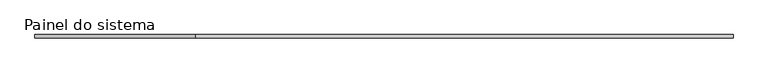
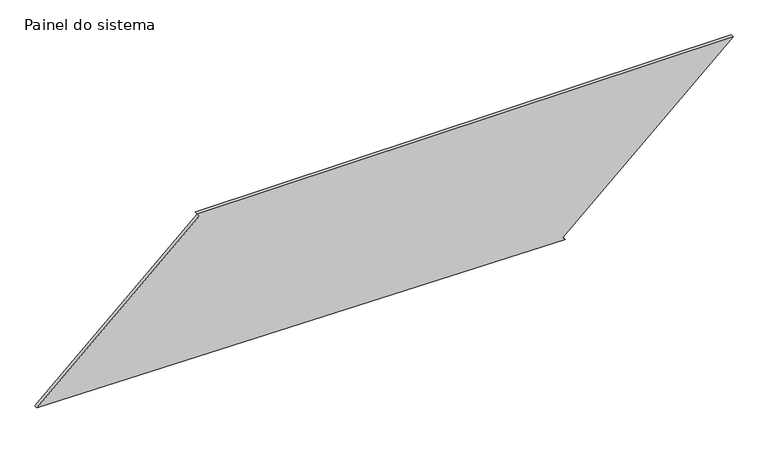
"""IFC4 building model written with IfcOpenShell, lengths in millimetres: plate geometry, Painel do sistema : Envidraçado."""

from ifc_helpers import new_model, si_unit, frame, origin, place, context, project, spatial, polyline, outline, extrude, source, transform, mapped, element, save


def painel_do_sistema_f254071a(model_context):
    return source(origin(), model_context, "Body", "SweptSolid", [
        extrude(outline(polyline([(0.0, 1281.7749259), (18.5968466, 1265.066925), (1106.0483241, 2475.4551949), (1106.0483241, -1336.534264), (1087.4514775, -1319.8262631), (49.1975382, -2475.4551949), (0.0, 1281.7749259)])), frame((0.0, 24.5, 0.0), z_axis=(0.0, 1.0, 0.0), x_axis=(0.0, 0.0, 1.0)), (0.0, 0.0, 1.0), 25.0),
    ])


if __name__ == "__main__":
    model = new_model("IFC4")
    model_context = context("Model", 3, world=origin())
    ifc_project = project(units=[si_unit("LENGTHUNIT", "METRE", prefix="MILLI")], contexts=[model_context])
    site = spatial("IfcSite", under=ifc_project)
    building = spatial("IfcBuilding", under=site)
    placement = place(None, origin())
    painel_do_sistema_shape = painel_do_sistema_f254071a(model_context)
    element("IfcPlate", 1, ObjectType="Painel do sistema : Envidraçado", at=placement, inside=building, context=model_context, shape_type="MappedRepresentation", body=[
        mapped(painel_do_sistema_shape, transform((0.0, 0.0, 0.0), x_axis=(1.0, 0.0, 0.0), y_axis=(0.0, 1.0, 0.0), z_axis=(0.0, 0.0, 1.0))),
    ])
    save(model, "model.ifc")

# Revit data of these elements
# Type "Painel do sistema : Envidraçado"
#   Construction Type Id = "GSP4R"
#   Analytic Construction = "Vidraça única Pilkington 1/8 pol"
#   Visual Light Transmittance = 0.9
#   Solar Heat Gain Coefficient = 0.86
#   Heat Transfer Coefficient (U) = 6.7069 W/(m²·K)
# Element 1 (IfcPlate, "Painel do sistema : Envidraçado")
#   Materials on its faces: "Vidro"
# Materials
#   "Vidro": class "Vidro", colour RGB 0 128 192, transparency 0.9, Description = "Vidro de sílica", Cost = 0
